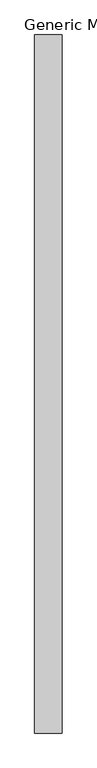
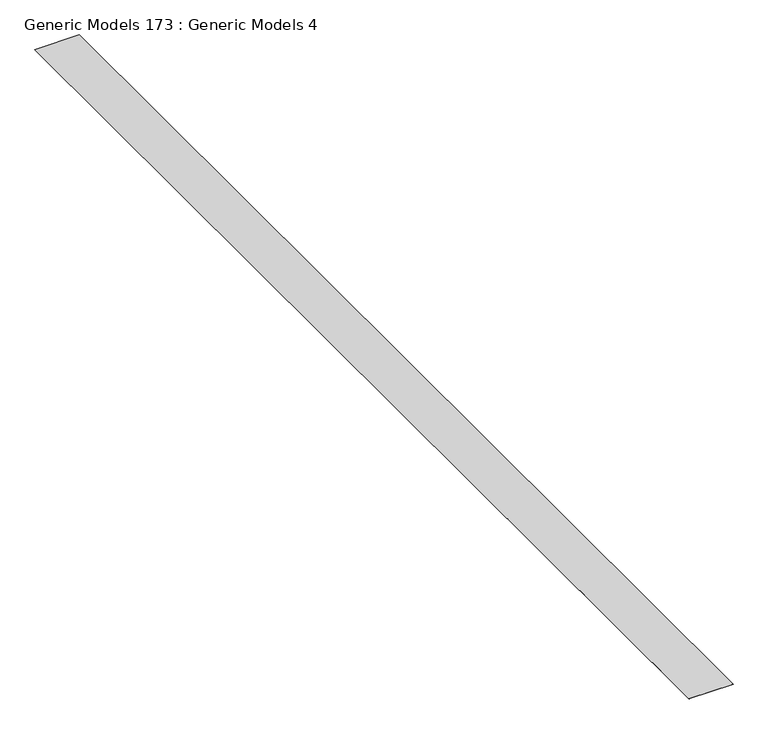
"""IFC4 building model written with IfcOpenShell, lengths in millimetres: proxy geometry, Generic Models 173 : Generic Models 4."""

from ifc_helpers import new_model, si_unit, frame, origin, place, context, project, spatial, polyline, outline, extrude, source, transform, mapped, element, save


def generic_models_173_generic_models_4_c01562a6(model_context):
    return source(origin(), model_context, "Body", "SweptSolid", [
        extrude(outline(polyline([(-5937.4236296, -5493.3230338), (-6426.3736296, -5493.3230338), (-6426.3736296, 7054.2769662), (-5937.4236296, 7054.2769662), (-5937.4236296, -5493.3230338)])), frame((0.0, 0.0, 123004.0085), z_axis=(0.0, 0.0, 1.0), x_axis=(1.0, 0.0, 0.0)), (0.0, 0.0, 1.0), 1.5875),
    ])


if __name__ == "__main__":
    model = new_model("IFC4")
    model_context = context("Model", 3, world=origin())
    ifc_project = project(units=[si_unit("LENGTHUNIT", "METRE", prefix="MILLI")], contexts=[model_context])
    site = spatial("IfcSite", under=ifc_project)
    building = spatial("IfcBuilding", under=site)
    placement = place(None, origin())
    generic_models_173_generic_models_4_shape = generic_models_173_generic_models_4_c01562a6(model_context)
    element("IfcBuildingElementProxy", 1, Name="Generic Models 173 : Generic Models 4", ObjectType="Generic Models 173 : Generic Models 4", at=placement, inside=building, context=model_context, shape_type="MappedRepresentation", body=[
        mapped(generic_models_173_generic_models_4_shape, transform((0.0, 0.0, 0.0), x_axis=(1.0, 0.0, 0.0), y_axis=(0.0, 1.0, 0.0), z_axis=(0.0, 0.0, 1.0))),
    ])
    save(model, "model.ifc")

# Revit data of these elements
# Element 1 (IfcBuildingElementProxy, "Generic Models 173 : Generic Models 4")
#   Materials on its faces: "_15 MIL VAPOR BARRIER"
# Materials
#   "_15 MIL VAPOR BARRIER": class "Generic", colour RGB 67 154 161, transparency 0, Cost = 0
